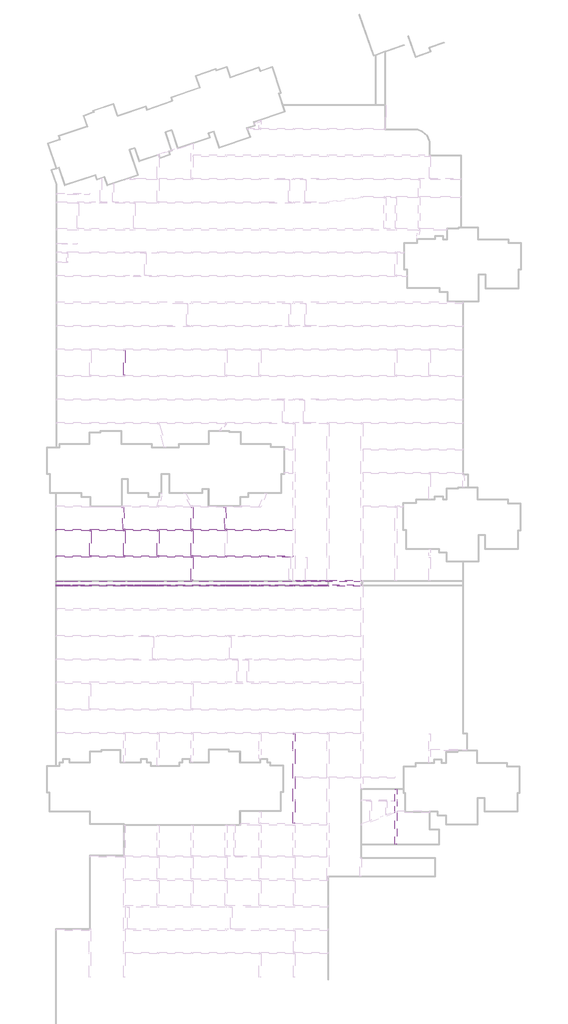
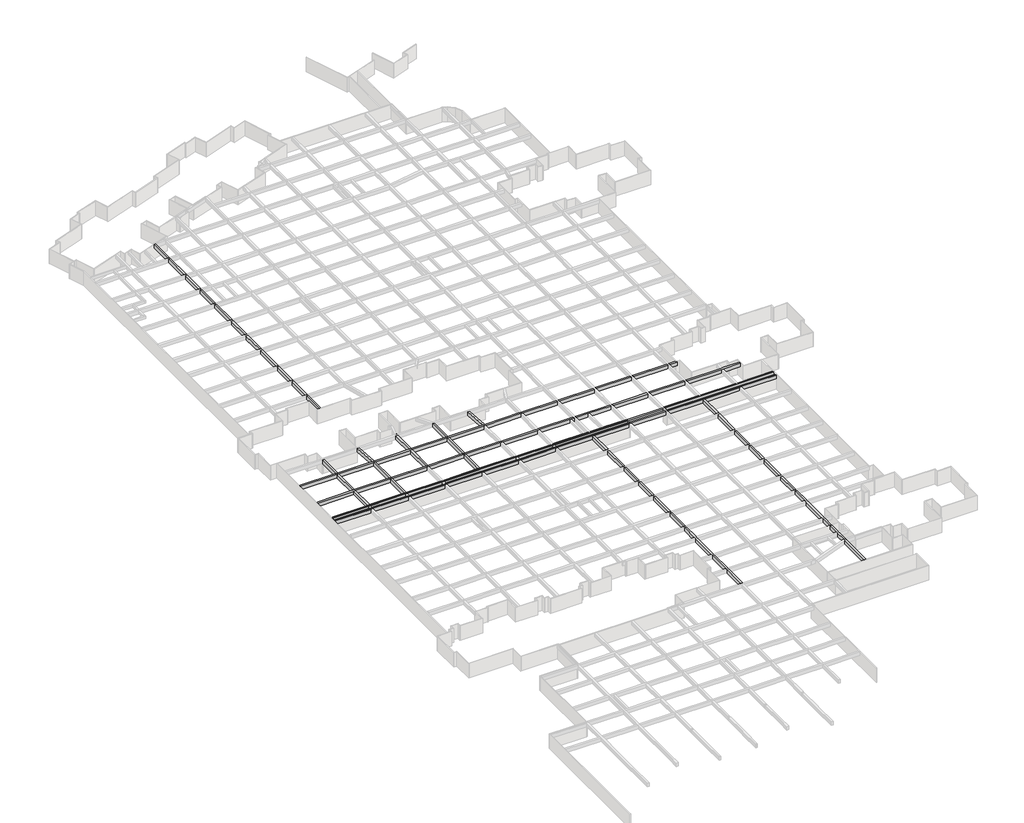
# One storey, part 10 of 14: 15 beams.
"""IFC4 building model written with IfcOpenShell, lengths in millimetres."""

from ifc_helpers import new_model, si_unit, frame, origin, place, context, project, spatial, polyline, outline, extrude, faceted_brep, element, save

model = new_model("IFC4")

# Units and contexts
model_context = context("Model", 3, world=origin())
ifc_project = project(units=[si_unit("LENGTHUNIT", "METRE", prefix="MILLI")], contexts=[model_context])

# Site, building, storey
site = spatial("IfcSite", under=ifc_project)
building = spatial("IfcBuilding", under=site)
storey = spatial("IfcBuildingStorey", under=building, Name="户型图", Elevation=0.0)

# Beams
placement = place(None, origin())
element("IfcBeam", 1, ObjectType="混凝土 - 矩形梁 : KL_beam", at=placement, inside=storey, context=model_context, shape_type="Brep", body=[
    faceted_brep([(-578267.6529954, -95855.8355501, 3300.0), (-577867.6529954, -95855.8355501, 3300.0), (-577867.6529954, -91159.4327531, 3300.0), (-578267.6529954, -91159.4327531, 3300.0), (-578267.6529954, -95855.8355501, 2500.0), (-578267.6529954, -91159.4327531, 2500.0), (-577867.6529954, -95855.8355501, 2500.0), (-577867.6529954, -91159.4327531, 2500.0)], [[[0, 1, 2, 3]], [[4, 0, 3, 5]], [[6, 4, 5, 7]], [[1, 6, 7, 2]], [[1, 0, 4, 6]], [[3, 2, 7, 5]]]),
    faceted_brep([(-578267.6529954, -33799.10215, 3300.0), (-577867.6529954, -33664.0771766, 3300.0), (-577867.6529954, -33664.0771766, 2500.0), (-578267.6529954, -33799.10215, 2500.0), (-577867.6529954, -38859.4327531, 3300.0), (-578267.6529954, -38859.4327531, 3300.0), (-578267.6529954, -38859.4327531, 2500.0), (-577867.6529954, -38859.4327531, 2500.0), (-577867.6529954, -33759.4327531, 3300.0), (-577867.6529954, -33759.4327531, 2500.0)], [[[0, 1, 2, 3]], [[4, 5, 6, 7]], [[1, 0, 5, 4, 8]], [[0, 3, 6, 5]], [[3, 2, 9, 7, 6]], [[2, 1, 8, 4, 7, 9]]]),
    faceted_brep([(-578267.6529954, -39259.4327531, 3300.0), (-577867.6529954, -39259.4327531, 3300.0), (-577867.6529954, -39259.4327531, 2500.0), (-578267.6529954, -39259.4327531, 2500.0), (-577867.6529954, -45159.4327531, 3300.0), (-578267.6529954, -45159.4327531, 3300.0), (-578267.6529954, -45159.4327531, 2500.0), (-577867.6529954, -45159.4327531, 2500.0)], [[[0, 1, 2, 3]], [[4, 5, 6, 7]], [[1, 0, 5, 4]], [[0, 3, 6, 5]], [[3, 2, 7, 6]], [[2, 1, 4, 7]]]),
    faceted_brep([(-578267.6529954, -45559.4327531, 3300.0), (-577867.6529954, -45559.4327531, 3300.0), (-577867.6529954, -45559.4327531, 2500.0), (-578267.6529954, -45559.4327531, 2500.0), (-577867.6529954, -50659.4327531, 3300.0), (-578267.6529954, -50659.4327531, 3300.0), (-578267.6529954, -50659.4327531, 2500.0), (-577867.6529954, -50659.4327531, 2500.0)], [[[0, 1, 2, 3]], [[4, 5, 6, 7]], [[1, 0, 5, 4]], [[0, 3, 6, 5]], [[3, 2, 7, 6]], [[2, 1, 4, 7]]]),
    faceted_brep([(-578267.6529954, -56559.4327531, 3300.0), (-577867.6529954, -56559.4327531, 3300.0), (-577867.6529954, -56559.4327531, 2500.0), (-578267.6529954, -56559.4327531, 2500.0), (-577867.6529954, -62459.4327531, 3300.0), (-578267.6529954, -62459.4327531, 3300.0), (-578267.6529954, -62459.4327531, 2500.0), (-577867.6529954, -62459.4327531, 2500.0)], [[[0, 1, 2, 3]], [[4, 5, 6, 7]], [[1, 0, 5, 4]], [[0, 3, 6, 5]], [[3, 2, 7, 6]], [[2, 1, 4, 7]]]),
    faceted_brep([(-577867.6529954, -56159.4327531, 3300.0), (-578267.6529954, -56159.4327531, 3300.0), (-578267.6529954, -56159.4327531, 2500.0), (-577867.6529954, -56159.4327531, 2500.0), (-577867.6529954, -51059.4327531, 3300.0), (-578267.6529954, -51059.4327531, 3300.0), (-578267.6529954, -51059.4327531, 2500.0), (-577867.6529954, -51059.4327531, 2500.0)], [[[0, 1, 2, 3]], [[1, 0, 4, 5]], [[2, 1, 5, 6]], [[3, 2, 6, 7]], [[0, 3, 7, 4]], [[5, 4, 7, 6]]]),
    faceted_brep([(-578267.6529954, -62859.4327531, 3300.0), (-577867.6529954, -62859.4327531, 3300.0), (-577867.6529954, -62859.4327531, 2500.0), (-578267.6529954, -62859.4327531, 2500.0), (-577867.6529954, -67959.4327531, 3300.0), (-578267.6529954, -67959.4327531, 3300.0), (-578267.6529954, -67959.4327531, 2500.0), (-577867.6529954, -67959.4327531, 2500.0)], [[[0, 1, 2, 3]], [[4, 5, 6, 7]], [[1, 0, 5, 4]], [[0, 3, 6, 5]], [[3, 2, 7, 6]], [[2, 1, 4, 7]]]),
    faceted_brep([(-578267.6529954, -68359.4327531, 3300.0), (-577867.6529954, -68359.4327531, 3300.0), (-577867.6529954, -68359.4327531, 2500.0), (-578267.6529954, -68359.4327531, 2500.0), (-577867.6529954, -73459.4327531, 3300.0), (-578267.6529954, -73459.4327531, 3300.0), (-578267.6529954, -73459.4327531, 2500.0), (-577867.6529954, -73459.4327531, 2500.0)], [[[0, 1, 2, 3]], [[4, 5, 6, 7]], [[1, 0, 5, 4]], [[0, 3, 6, 5]], [[3, 2, 7, 6]], [[2, 1, 4, 7]]]),
    faceted_brep([(-578267.6529954, -73859.4327531, 3300.0), (-577867.6529954, -73859.4327531, 3300.0), (-577867.6529954, -73859.4327531, 2500.0), (-578267.6529954, -73859.4327531, 2500.0), (-577867.6529954, -79759.4327531, 3300.0), (-578267.6529954, -79759.4327531, 3300.0), (-578267.6529954, -79759.4327531, 2500.0), (-577867.6529954, -79759.4327531, 2500.0)], [[[0, 1, 2, 3]], [[4, 5, 6, 7]], [[1, 0, 5, 4]], [[0, 3, 6, 5]], [[3, 2, 7, 6]], [[2, 1, 4, 7]]]),
    faceted_brep([(-578267.6529954, -80159.4327531, 3300.0), (-577867.6529954, -80159.4327531, 3300.0), (-577867.6529954, -80159.4327531, 2500.0), (-578267.6529954, -80159.4327531, 2500.0), (-577867.6529954, -85259.4327531, 3300.0), (-578267.6529954, -85259.4327531, 3300.0), (-578267.6529954, -85259.4327531, 2500.0), (-577867.6529954, -85259.4327531, 2500.0)], [[[0, 1, 2, 3]], [[4, 5, 6, 7]], [[1, 0, 5, 4]], [[0, 3, 6, 5]], [[3, 2, 7, 6]], [[2, 1, 4, 7]]]),
    faceted_brep([(-578267.6529954, -85659.4327531, 3300.0), (-577867.6529954, -85659.4327531, 3300.0), (-577867.6529954, -85659.4327531, 2500.0), (-578267.6529954, -85659.4327531, 2500.0), (-577867.6529954, -90759.4327531, 3300.0), (-578267.6529954, -90759.4327531, 3300.0), (-578267.6529954, -90759.4327531, 2500.0), (-577867.6529954, -90759.4327531, 2500.0)], [[[0, 1, 2, 3]], [[4, 5, 6, 7]], [[1, 0, 5, 4]], [[0, 3, 6, 5]], [[3, 2, 7, 6]], [[2, 1, 4, 7]]]),
])
element("IfcBeam", 2, ObjectType="混凝土 - 矩形梁 : KL_beam", at=placement, inside=storey, context=model_context, shape_type="Brep", body=[
    faceted_brep([(-512410.8523761, -116217.5126628, 3300.0), (-512410.8523761, -116097.5126628, 3300.0), (-512410.8523761, -115957.5126628, 3300.0), (-513867.6529954, -115957.5126628, 3300.0), (-513867.6529954, -116357.5126628, 3300.0), (-512290.8523761, -116357.5126628, 3300.0), (-512290.8523761, -116217.5126628, 3300.0), (-512410.8523761, -115957.5126628, 2500.0), (-513867.6529954, -115957.5126628, 2500.0), (-512410.8523761, -116217.5126628, 2500.0), (-512290.8523761, -116217.5126628, 2500.0), (-512290.8523761, -116357.5126628, 2500.0), (-513867.6529954, -116357.5126628, 2500.0)], [[[0, 1, 2, 3, 4, 5, 6]], [[2, 7, 8, 3]], [[7, 9, 10, 11, 12, 8]], [[11, 5, 4, 12]], [[5, 11, 10, 6]], [[0, 9, 7, 2, 1]], [[4, 3, 8, 12]], [[9, 0, 6, 10]]]),
    faceted_brep([(-594137.5937933, -116357.5126628, 3300.0), (-594137.5937933, -115957.5126628, 3300.0), (-594137.5937933, -115957.5126628, 2500.0), (-594137.5937933, -116357.5126628, 2500.0), (-538267.6529954, -115957.5126628, 3300.0), (-538267.6529954, -116357.5126628, 3300.0), (-538267.6529954, -116357.5126628, 2500.0), (-538267.6529954, -115957.5126628, 2500.0), (-586231.2602569, -116357.5126628, 3300.0), (-585831.2602569, -116357.5126628, 3300.0), (-578267.6529954, -116357.5126628, 3300.0), (-577867.6529954, -116357.5126628, 3300.0), (-570267.6529954, -116357.5126628, 3300.0), (-569867.6529954, -116357.5126628, 3300.0), (-562267.6529954, -116357.5126628, 3300.0), (-561867.6529954, -116357.5126628, 3300.0), (-554267.6529954, -116357.5126628, 3300.0), (-553867.6529954, -116357.5126628, 3300.0), (-546267.6529954, -116357.5126628, 3300.0), (-545867.6529954, -116357.5126628, 3300.0), (-545867.6529954, -115957.5126628, 3300.0), (-546267.6529954, -115957.5126628, 3300.0), (-553881.1620009, -115957.5126628, 3300.0), (-554282.1387601, -115957.5126628, 3300.0), (-561867.6529954, -115957.5126628, 3300.0), (-562267.6529954, -115957.5126628, 3300.0), (-569867.6529954, -115957.5126628, 3300.0), (-570267.6529954, -115957.5126628, 3300.0), (-577881.1499782, -115957.5126628, 3300.0), (-578282.1267374, -115957.5126628, 3300.0), (-585831.2602569, -115957.5126628, 3300.0), (-586231.2602569, -115957.5126628, 3300.0), (-545867.6529954, -115957.5126628, 2500.0), (-546267.6529954, -115957.5126628, 2500.0), (-553881.1620009, -115957.5126628, 2500.0), (-554282.1387601, -115957.5126628, 2500.0), (-561867.6529954, -115957.5126628, 2500.0), (-562267.6529954, -115957.5126628, 2500.0), (-569867.6529954, -115957.5126628, 2500.0), (-570267.6529954, -115957.5126628, 2500.0), (-577881.1499782, -115957.5126628, 2500.0), (-578282.1267374, -115957.5126628, 2500.0), (-585831.2602569, -115957.5126628, 2500.0), (-586231.2602569, -115957.5126628, 2500.0), (-545867.6529954, -116357.5126628, 2500.0), (-546267.6529954, -116357.5126628, 2500.0), (-553867.6529954, -116357.5126628, 2500.0), (-554267.6529954, -116357.5126628, 2500.0), (-561867.6529954, -116357.5126628, 2500.0), (-562267.6529954, -116357.5126628, 2500.0), (-569867.6529954, -116357.5126628, 2500.0), (-570267.6529954, -116357.5126628, 2500.0), (-577867.6529954, -116357.5126628, 2500.0), (-578267.6529954, -116357.5126628, 2500.0), (-585831.2602569, -116357.5126628, 2500.0), (-586231.2602569, -116357.5126628, 2500.0)], [[[0, 1, 2, 3]], [[4, 5, 6, 7]], [[1, 0, 8, 9, 10, 11, 12, 13, 14, 15, 16, 17, 18, 19, 5, 4, 20, 21, 22, 23, 24, 25, 26, 27, 28, 29, 30, 31]], [[2, 1, 31, 30, 29, 28, 27, 26, 25, 24, 23, 22, 21, 20, 4, 7, 32, 33, 34, 35, 36, 37, 38, 39, 40, 41, 42, 43]], [[3, 2, 43, 42, 41, 40, 39, 38, 37, 36, 35, 34, 33, 32, 7, 6, 44, 45, 46, 47, 48, 49, 50, 51, 52, 53, 54, 55]], [[0, 3, 55, 54, 53, 52, 51, 50, 49, 48, 47, 46, 45, 44, 6, 5, 19, 18, 17, 16, 15, 14, 13, 12, 11, 10, 9, 8]]]),
    faceted_brep([(-537867.6529954, -116357.5126628, 3300.0), (-537867.6529954, -115957.5126628, 3300.0), (-537867.6529954, -115957.5126628, 2500.0), (-537867.6529954, -116357.5126628, 2500.0), (-530267.6529954, -115957.5126628, 3300.0), (-530267.6529954, -116357.5126628, 3300.0), (-530267.6529954, -116357.5126628, 2500.0), (-530267.6529954, -115957.5126628, 2500.0)], [[[0, 1, 2, 3]], [[4, 5, 6, 7]], [[1, 0, 5, 4]], [[2, 1, 4, 7]], [[3, 2, 7, 6]], [[0, 3, 6, 5]]]),
    faceted_brep([(-529867.6529954, -116357.5126628, 3300.0), (-529867.6529954, -115957.5126628, 3300.0), (-529867.6529954, -115957.5126628, 2500.0), (-529867.6529954, -116357.5126628, 2500.0), (-522267.6529954, -115957.5126628, 3300.0), (-522267.6529954, -116357.5126628, 3300.0), (-522267.6529954, -116357.5126628, 2500.0), (-522267.6529954, -115957.5126628, 2500.0)], [[[0, 1, 2, 3]], [[4, 5, 6, 7]], [[1, 0, 5, 4]], [[2, 1, 4, 7]], [[3, 2, 7, 6]], [[0, 3, 6, 5]]]),
    faceted_brep([(-521867.6529954, -116357.5126628, 3300.0), (-521867.6529954, -115957.5126628, 3300.0), (-521867.6529954, -115957.5126628, 2500.0), (-521867.6529954, -116357.5126628, 2500.0), (-514267.6529954, -115957.5126628, 3300.0), (-514267.6529954, -116357.5126628, 3300.0), (-514267.6529954, -116357.5126628, 2500.0), (-514267.6529954, -115957.5126628, 2500.0)], [[[0, 1, 2, 3]], [[4, 5, 6, 7]], [[1, 0, 5, 4]], [[2, 1, 4, 7]], [[3, 2, 7, 6]], [[0, 3, 6, 5]]]),
])
element("IfcBeam", 3, ObjectType="混凝土 - 矩形梁 : KL_beam", at=placement, inside=storey, context=model_context, shape_type="Brep", body=[
    faceted_brep([(-594137.5937933, -122259.4327531, 3300.0), (-594137.5937933, -122659.4327531, 3300.0), (-586231.2602569, -122659.4327531, 3300.0), (-585831.2602569, -122659.4327531, 3300.0), (-578267.6529954, -122659.4327531, 3300.0), (-577867.6529954, -122659.4327531, 3300.0), (-570267.6529954, -122659.4327531, 3300.0), (-569867.6529954, -122659.4327531, 3300.0), (-562267.6529954, -122659.4327531, 3300.0), (-561867.6529954, -122659.4327531, 3300.0), (-554267.6529954, -122659.4327531, 3300.0), (-553867.6529954, -122659.4327531, 3300.0), (-546267.6529954, -122659.4327531, 3300.0), (-545867.6529954, -122659.4327531, 3300.0), (-539217.6529954, -122659.4327531, 3300.0), (-538917.6529954, -122659.4327531, 3300.0), (-538267.6529954, -122659.4327531, 3300.0), (-538267.6529954, -122259.4327531, 3300.0), (-545867.6529954, -122259.4327531, 3300.0), (-546267.6529954, -122259.4327531, 3300.0), (-553867.6529954, -122259.4327531, 3300.0), (-554267.6529954, -122259.4327531, 3300.0), (-561867.6529954, -122259.4327531, 3300.0), (-562267.6529954, -122259.4327531, 3300.0), (-569867.6529954, -122259.4327531, 3300.0), (-570267.6529954, -122259.4327531, 3300.0), (-577867.6529954, -122259.4327531, 3300.0), (-578267.6529954, -122259.4327531, 3300.0), (-585831.2602569, -122259.4327531, 3300.0), (-586231.2602569, -122259.4327531, 3300.0), (-594137.5937933, -122659.4327531, 2500.0), (-586231.2602569, -122659.4327531, 2500.0), (-585831.2602569, -122659.4327531, 2500.0), (-578267.6529954, -122659.4327531, 2500.0), (-577867.6529954, -122659.4327531, 2500.0), (-570267.6529954, -122659.4327531, 2500.0), (-569867.6529954, -122659.4327531, 2500.0), (-562267.6529954, -122659.4327531, 2500.0), (-561867.6529954, -122659.4327531, 2500.0), (-554267.6529954, -122659.4327531, 2500.0), (-553867.6529954, -122659.4327531, 2500.0), (-546267.6529954, -122659.4327531, 2500.0), (-545867.6529954, -122659.4327531, 2500.0), (-538267.6529954, -122659.4327531, 2500.0), (-594137.5937933, -122259.4327531, 2500.0), (-586231.2602569, -122259.4327531, 2500.0), (-585831.2602569, -122259.4327531, 2500.0), (-578267.6529954, -122259.4327531, 2500.0), (-577867.6529954, -122259.4327531, 2500.0), (-570267.6529954, -122259.4327531, 2500.0), (-569867.6529954, -122259.4327531, 2500.0), (-562267.6529954, -122259.4327531, 2500.0), (-561867.6529954, -122259.4327531, 2500.0), (-554267.6529954, -122259.4327531, 2500.0), (-553867.6529954, -122259.4327531, 2500.0), (-546267.6529954, -122259.4327531, 2500.0), (-545867.6529954, -122259.4327531, 2500.0), (-538267.6529954, -122259.4327531, 2500.0)], [[[0, 1, 2, 3, 4, 5, 6, 7, 8, 9, 10, 11, 12, 13, 14, 15, 16, 17, 18, 19, 20, 21, 22, 23, 24, 25, 26, 27, 28, 29]], [[1, 30, 31, 32, 33, 34, 35, 36, 37, 38, 39, 40, 41, 42, 43, 16, 15, 14, 13, 12, 11, 10, 9, 8, 7, 6, 5, 4, 3, 2]], [[30, 44, 45, 46, 47, 48, 49, 50, 51, 52, 53, 54, 55, 56, 57, 43, 42, 41, 40, 39, 38, 37, 36, 35, 34, 33, 32, 31]], [[44, 0, 29, 28, 27, 26, 25, 24, 23, 22, 21, 20, 19, 18, 17, 57, 56, 55, 54, 53, 52, 51, 50, 49, 48, 47, 46, 45]], [[1, 0, 44, 30]], [[17, 16, 43, 57]]]),
    faceted_brep([(-502127.6529954, -122259.4327531, 3300.0), (-502127.6529954, -122659.4327531, 3300.0), (-502127.6529954, -122659.4327531, 2500.0), (-502127.6529954, -122259.4327531, 2500.0), (-505867.6529954, -122259.4327531, 3300.0), (-506267.6529954, -122259.4327531, 3300.0), (-513867.6529954, -122259.4327531, 3300.0), (-513867.6529954, -122659.4327531, 3300.0), (-506267.6529954, -122659.4327531, 3300.0), (-505867.6529954, -122659.4327531, 3300.0), (-513867.6529954, -122659.4327531, 2500.0), (-506267.6529954, -122659.4327531, 2500.0), (-505867.6529954, -122659.4327531, 2500.0), (-513867.6529954, -122259.4327531, 2500.0), (-506267.6529954, -122259.4327531, 2500.0), (-505867.6529954, -122259.4327531, 2500.0)], [[[0, 1, 2, 3]], [[1, 0, 4, 5, 6, 7, 8, 9]], [[2, 1, 9, 8, 7, 10, 11, 12]], [[3, 2, 12, 11, 10, 13, 14, 15]], [[0, 3, 15, 14, 13, 6, 5, 4]], [[7, 6, 13, 10]]]),
    faceted_brep([(-537867.6529954, -122659.4327531, 3300.0), (-537867.6529954, -122259.4327531, 3300.0), (-537867.6529954, -122259.4327531, 2500.0), (-537867.6529954, -122659.4327531, 2500.0), (-530267.6529954, -122259.4327531, 3300.0), (-530267.6529954, -122659.4327531, 3300.0), (-530267.6529954, -122659.4327531, 2500.0), (-530267.6529954, -122259.4327531, 2500.0), (-535317.6529954, -122659.4327531, 3300.0), (-535017.6529954, -122659.4327531, 3300.0)], [[[0, 1, 2, 3]], [[4, 5, 6, 7]], [[1, 0, 8, 9, 5, 4]], [[0, 3, 6, 5, 9, 8]], [[3, 2, 7, 6]], [[2, 1, 4, 7]]]),
    faceted_brep([(-529867.6529954, -122259.4327531, 3300.0), (-529867.6529954, -122659.4327531, 3300.0), (-522267.6529954, -122659.4327531, 3300.0), (-522267.6529954, -122259.4327531, 3300.0), (-529867.6529954, -122659.4327531, 2500.0), (-522267.6529954, -122659.4327531, 2500.0), (-529867.6529954, -122259.4327531, 2500.0), (-522267.6529954, -122259.4327531, 2500.0)], [[[0, 1, 2, 3]], [[1, 4, 5, 2]], [[4, 6, 7, 5]], [[6, 0, 3, 7]], [[1, 0, 6, 4]], [[3, 2, 5, 7]]]),
    faceted_brep([(-521867.6529954, -122659.4327531, 3300.0), (-521867.6529954, -122259.4327531, 3300.0), (-521867.6529954, -122259.4327531, 2500.0), (-521867.6529954, -122659.4327531, 2500.0), (-514267.6529954, -122259.4327531, 3300.0), (-514267.6529954, -122659.4327531, 3300.0), (-514267.6529954, -122659.4327531, 2500.0), (-514267.6529954, -122259.4327531, 2500.0)], [[[0, 1, 2, 3]], [[4, 5, 6, 7]], [[1, 0, 5, 4]], [[0, 3, 6, 5]], [[3, 2, 7, 6]], [[2, 1, 4, 7]]]),
])
element("IfcBeam", 4, ObjectType="混凝土 - 矩形梁 : KL_beam", at=placement, inside=storey, context=model_context, shape_type="Brep", body=[
    faceted_brep([(-521867.6529954, -128359.4327532, 3300.0), (-498227.6529954, -128359.4327532, 3300.0), (-498227.6529954, -128219.4327532, 3300.0), (-521867.6529954, -128219.4327532, 3300.0), (-498227.6529954, -128359.4327532, 2500.0), (-521867.6529954, -128359.4327532, 2500.0), (-498227.6529954, -128219.4327532, 2500.0), (-521867.6529954, -128219.4327532, 2500.0)], [[[0, 1, 2, 3]], [[4, 1, 0, 5]], [[2, 6, 7, 3]], [[4, 5, 7, 6]], [[1, 4, 6, 2]], [[5, 0, 3, 7]]]),
    faceted_brep([(-498227.6529954, -127959.4327532, 3300.0), (-498227.6529954, -127959.4327532, 2500.0), (-505867.6529954, -127959.4327532, 2500.0), (-505867.6529954, -127959.4327532, 3300.0), (-498227.6529954, -128099.4327532, 3300.0), (-498227.6529954, -128099.4327532, 2500.0), (-505867.6529954, -128099.4327532, 2500.0), (-505867.6529954, -128099.4327532, 3300.0)], [[[0, 1, 2, 3]], [[1, 0, 4, 5]], [[3, 2, 6, 7]], [[4, 7, 6, 5]], [[0, 3, 7, 4]], [[2, 1, 5, 6]]]),
    faceted_brep([(-521867.6529954, -127959.4327532, 2500.0), (-514267.6529954, -127959.4327532, 2500.0), (-514267.6529954, -128099.4327532, 2500.0), (-521867.6529954, -128099.4327532, 2500.0), (-521867.6529954, -127959.4327532, 3300.0), (-521867.6529954, -128099.4327532, 3300.0), (-514267.6529954, -127959.4327532, 3300.0), (-514267.6529954, -128099.4327532, 3300.0)], [[[0, 1, 2, 3]], [[4, 0, 3, 5]], [[1, 6, 7, 2]], [[0, 4, 6, 1]], [[6, 4, 5, 7]], [[7, 5, 3, 2]]]),
    faceted_brep([(-594137.5937933, -128359.4327532, 2500.0), (-594137.5937933, -128359.4327532, 3300.0), (-594137.5937933, -128219.4327532, 3300.0), (-594137.5937933, -128219.4327532, 2500.0), (-537867.6529954, -127959.4327532, 3300.0), (-537867.6529954, -127959.4327532, 2500.0), (-537867.6529954, -128099.4327532, 2500.0), (-537867.6529954, -128099.4327532, 3300.0), (-530067.6731545, -128219.4327532, 3300.0), (-530067.6731545, -128219.4327532, 2500.0), (-522267.6529954, -127959.4327532, 3300.0), (-522267.6529954, -128359.4327532, 3300.0), (-522267.6529954, -128359.4327532, 2500.0), (-522267.6529954, -127959.4327532, 2500.0), (-586331.2602569, -128359.4327532, 3300.0), (-585931.2602569, -128359.4327532, 3300.0), (-578267.6529954, -128359.4327532, 3300.0), (-577867.6529954, -128359.4327532, 3300.0), (-570267.6529954, -128359.4327532, 3300.0), (-569867.6529954, -128359.4327532, 3300.0), (-554267.6529954, -128359.4327532, 3300.0), (-553867.6529954, -128359.4327532, 3300.0), (-546267.6529954, -128359.4327532, 3300.0), (-545867.6529954, -128359.4327532, 3300.0), (-529867.6529954, -127959.4327532, 3300.0), (-530267.6529954, -127959.4327532, 3300.0), (-535017.6529954, -127959.4327532, 3300.0), (-535317.6529954, -127959.4327532, 3300.0), (-530067.6731545, -128099.4327532, 3300.0), (-529867.6529954, -127959.4327532, 2500.0), (-530267.6529954, -127959.4327532, 2500.0), (-586331.2602569, -128359.4327532, 2500.0), (-585931.2602569, -128359.4327532, 2500.0), (-578267.6529954, -128359.4327532, 2500.0), (-577867.6529954, -128359.4327532, 2500.0), (-570267.6529954, -128359.4327532, 2500.0), (-569867.6529954, -128359.4327532, 2500.0), (-554267.6529954, -128359.4327532, 2500.0), (-553867.6529954, -128359.4327532, 2500.0), (-546267.6529954, -128359.4327532, 2500.0), (-545867.6529954, -128359.4327532, 2500.0), (-530067.6731545, -128099.4327532, 2500.0)], [[[0, 1, 2, 3]], [[4, 5, 6, 7]], [[8, 9, 3, 2]], [[10, 11, 12, 13]], [[1, 14, 15, 16, 17, 18, 19, 20, 21, 22, 23, 11, 10, 24, 25, 26, 27, 4, 7, 28, 8, 2]], [[5, 4, 27, 26, 25, 24, 10, 13, 29, 30]], [[1, 0, 31, 32, 33, 34, 35, 36, 37, 38, 39, 40, 12, 11, 23, 22, 21, 20, 19, 18, 17, 16, 15, 14]], [[41, 28, 7, 6]], [[9, 8, 28, 41]], [[5, 30, 29, 13, 12, 40, 39, 38, 37, 36, 35, 34, 33, 32, 31, 0, 3, 9, 41, 6]]]),
    faceted_brep([(-538267.6529954, -127959.4327532, 2500.0), (-538267.6529954, -127959.4327532, 3300.0), (-538267.6529954, -128099.4327532, 3300.0), (-538267.6529954, -128099.4327532, 2500.0), (-594137.5937933, -127959.4327532, 2500.0), (-594137.5937933, -127959.4327532, 3300.0), (-586231.2602569, -127959.4327532, 3300.0), (-585831.2602569, -127959.4327532, 3300.0), (-578267.6529954, -127959.4327532, 3300.0), (-577867.6529954, -127959.4327532, 3300.0), (-570267.6529954, -127959.4327532, 3300.0), (-569867.6529954, -127959.4327532, 3300.0), (-562267.6529954, -127959.4327532, 3300.0), (-561867.6529954, -127959.4327532, 3300.0), (-554267.6529954, -127959.4327532, 3300.0), (-553867.6529954, -127959.4327532, 3300.0), (-546267.6529954, -127959.4327532, 3300.0), (-545867.6529954, -127959.4327532, 3300.0), (-545867.6529954, -127959.4327532, 2500.0), (-546267.6529954, -127959.4327532, 2500.0), (-553867.6529954, -127959.4327532, 2500.0), (-554267.6529954, -127959.4327532, 2500.0), (-561867.6529954, -127959.4327532, 2500.0), (-562267.6529954, -127959.4327532, 2500.0), (-569867.6529954, -127959.4327532, 2500.0), (-570267.6529954, -127959.4327532, 2500.0), (-577867.6529954, -127959.4327532, 2500.0), (-578267.6529954, -127959.4327532, 2500.0), (-585831.2602569, -127959.4327532, 2500.0), (-586231.2602569, -127959.4327532, 2500.0), (-594137.5937933, -128099.4327532, 2500.0), (-594137.5937933, -128099.4327532, 3300.0)], [[[0, 1, 2, 3]], [[4, 5, 6, 7, 8, 9, 10, 11, 12, 13, 14, 15, 16, 17, 1, 0, 18, 19, 20, 21, 22, 23, 24, 25, 26, 27, 28, 29]], [[4, 29, 28, 27, 26, 25, 24, 23, 22, 21, 20, 19, 18, 0, 3, 30]], [[5, 4, 30, 31]], [[1, 17, 16, 15, 14, 13, 12, 11, 10, 9, 8, 7, 6, 5, 31, 2]], [[31, 30, 3, 2]]]),
    faceted_brep([(-513867.6529954, -127959.4327532, 3300.0), (-513867.6529954, -127959.4327532, 2500.0), (-513867.6529954, -128099.4327532, 2500.0), (-513867.6529954, -128099.4327532, 3300.0), (-506267.6529954, -127959.4327532, 2500.0), (-506267.6529954, -127959.4327532, 3300.0), (-506267.6529954, -128099.4327532, 3300.0), (-506267.6529954, -128099.4327532, 2500.0)], [[[0, 1, 2, 3]], [[4, 5, 6, 7]], [[1, 0, 5, 4]], [[5, 0, 3, 6]], [[1, 4, 7, 2]], [[6, 3, 2, 7]]]),
])
element("IfcBeam", 5, ObjectType="混凝土 - 矩形梁 : KL_beam", at=placement, inside=storey, context=model_context, shape_type="Brep", body=[
    faceted_brep([(-522267.6529954, -129034.4327531, 3300.0), (-545867.6529954, -129034.4327531, 3300.0), (-546267.6529954, -129034.4327531, 3300.0), (-553867.6529954, -129034.4327531, 3300.0), (-554267.6529954, -129034.4327531, 3300.0), (-569867.6529954, -129034.4327531, 3300.0), (-570267.6529954, -129034.4327531, 3300.0), (-577867.6529954, -129034.4327531, 3300.0), (-578267.6529954, -129034.4327531, 3300.0), (-585931.2602569, -129034.4327531, 3300.0), (-586331.2602569, -129034.4327531, 3300.0), (-594137.5937933, -129034.4327531, 3300.0), (-594137.5937933, -129174.4327531, 3300.0), (-530067.6731545, -129174.4327531, 3300.0), (-530067.6731545, -129294.4327531, 3300.0), (-594137.5937933, -129294.4327531, 3300.0), (-594137.5937933, -129434.4327531, 3300.0), (-586331.2602569, -129434.4327531, 3300.0), (-585931.2602569, -129434.4327531, 3300.0), (-578267.6529954, -129434.4327531, 3300.0), (-577867.6529954, -129434.4327531, 3300.0), (-570267.6529954, -129434.4327531, 3300.0), (-569867.6529954, -129434.4327531, 3300.0), (-562267.6529954, -129434.4327531, 3300.0), (-561867.6529954, -129434.4327531, 3300.0), (-554267.6529954, -129434.4327531, 3300.0), (-553867.6529954, -129434.4327531, 3300.0), (-546267.6529954, -129434.4327531, 3300.0), (-545867.6529954, -129434.4327531, 3300.0), (-538267.6529954, -129434.4327531, 3300.0), (-537867.6529954, -129434.4327531, 3300.0), (-530267.6529954, -129434.4327531, 3300.0), (-529867.6529954, -129434.4327531, 3300.0), (-522267.6529954, -129434.4327531, 3300.0), (-594137.5937933, -129434.4327531, 2500.0), (-586331.2602569, -129434.4327531, 2500.0), (-585931.2602569, -129434.4327531, 2500.0), (-578267.6529954, -129434.4327531, 2500.0), (-577867.6529954, -129434.4327531, 2500.0), (-570267.6529954, -129434.4327531, 2500.0), (-569867.6529954, -129434.4327531, 2500.0), (-562267.6529954, -129434.4327531, 2500.0), (-561867.6529954, -129434.4327531, 2500.0), (-554267.6529954, -129434.4327531, 2500.0), (-553867.6529954, -129434.4327531, 2500.0), (-546267.6529954, -129434.4327531, 2500.0), (-545867.6529954, -129434.4327531, 2500.0), (-538267.6529954, -129434.4327531, 2500.0), (-537867.6529954, -129434.4327531, 2500.0), (-530267.6529954, -129434.4327531, 2500.0), (-529867.6529954, -129434.4327531, 2500.0), (-522267.6529954, -129434.4327531, 2500.0), (-594137.5937933, -129294.4327531, 2500.0), (-530067.6731545, -129294.4327531, 2500.0), (-530067.6731545, -129174.4327531, 2500.0), (-594137.5937933, -129174.4327531, 2500.0), (-594137.5937933, -129034.4327531, 2500.0), (-586331.2602569, -129034.4327531, 2500.0), (-585931.2602569, -129034.4327531, 2500.0), (-578267.6529954, -129034.4327531, 2500.0), (-577867.6529954, -129034.4327531, 2500.0), (-570267.6529954, -129034.4327531, 2500.0), (-569867.6529954, -129034.4327531, 2500.0), (-554267.6529954, -129034.4327531, 2500.0), (-553867.6529954, -129034.4327531, 2500.0), (-546267.6529954, -129034.4327531, 2500.0), (-545867.6529954, -129034.4327531, 2500.0), (-522267.6529954, -129034.4327531, 2500.0)], [[[0, 1, 2, 3, 4, 5, 6, 7, 8, 9, 10, 11, 12, 13, 14, 15, 16, 17, 18, 19, 20, 21, 22, 23, 24, 25, 26, 27, 28, 29, 30, 31, 32, 33]], [[16, 34, 35, 36, 37, 38, 39, 40, 41, 42, 43, 44, 45, 46, 47, 48, 49, 50, 51, 33, 32, 31, 30, 29, 28, 27, 26, 25, 24, 23, 22, 21, 20, 19, 18, 17]], [[51, 50, 49, 48, 47, 46, 45, 44, 43, 42, 41, 40, 39, 38, 37, 36, 35, 34, 52, 53, 54, 55, 56, 57, 58, 59, 60, 61, 62, 63, 64, 65, 66, 67]], [[56, 11, 10, 9, 8, 7, 6, 5, 4, 3, 2, 1, 0, 67, 66, 65, 64, 63, 62, 61, 60, 59, 58, 57]], [[34, 16, 15, 52]], [[0, 33, 51, 67]], [[54, 13, 12, 55]], [[14, 53, 52, 15]], [[13, 54, 53, 14]], [[11, 56, 55, 12]]]),
    faceted_brep([(-498227.6529954, -129034.4327531, 2500.0), (-498227.6529954, -129034.4327531, 3300.0), (-498227.6529954, -129174.4327531, 3300.0), (-498227.6529954, -129174.4327531, 2500.0), (-521867.6529954, -129034.4327531, 3300.0), (-521867.6529954, -129174.4327531, 3300.0), (-521867.6529954, -129034.4327531, 2500.0), (-521867.6529954, -129174.4327531, 2500.0)], [[[0, 1, 2, 3]], [[1, 4, 5, 2]], [[1, 0, 6, 4]], [[3, 2, 5, 7]], [[4, 6, 7, 5]], [[6, 0, 3, 7]]]),
    faceted_brep([(-521867.6529954, -129434.4327531, 2500.0), (-521867.6529954, -129434.4327531, 3300.0), (-521867.6529954, -129294.4327531, 3300.0), (-521867.6529954, -129294.4327531, 2500.0), (-498227.6529954, -129434.4327531, 2500.0), (-498227.6529954, -129434.4327531, 3300.0), (-505867.6529954, -129434.4327531, 3300.0), (-506267.6529954, -129434.4327531, 3300.0), (-513867.6529954, -129434.4327531, 3300.0), (-514267.6529954, -129434.4327531, 3300.0), (-514267.6529954, -129434.4327531, 2500.0), (-513867.6529954, -129434.4327531, 2500.0), (-506267.6529954, -129434.4327531, 2500.0), (-505867.6529954, -129434.4327531, 2500.0), (-498227.6529954, -129294.4327531, 2500.0), (-498227.6529954, -129294.4327531, 3300.0)], [[[0, 1, 2, 3]], [[4, 5, 6, 7, 8, 9, 1, 0, 10, 11, 12, 13]], [[4, 13, 12, 11, 10, 0, 3, 14]], [[15, 14, 3, 2]], [[5, 4, 14, 15]], [[1, 9, 8, 7, 6, 5, 15, 2]]]),
])
element("IfcBeam", 6, ObjectType="混凝土 - 矩形梁 : KL_beam", at=placement, inside=storey, context=model_context, shape_type="SweptSolid", body=[
    extrude(outline(polyline([(-553881.1620009, -115957.5126628), (-554282.1387601, -115957.5126628), (-554638.6312353, -110859.4327531), (-554237.654476, -110859.4327531), (-553881.1620009, -115957.5126628)])), frame((0.0, 0.0, 2500.0), z_axis=(0.0, 0.0, 1.0), x_axis=(1.0, 0.0, 0.0)), (0.0, 0.0, 1.0), 800.0),
])
element("IfcBeam", 7, ObjectType="混凝土 - 矩形梁 : KL_beam", at=placement, inside=storey, context=model_context, shape_type="SweptSolid", body=[
    extrude(outline(polyline([(-562267.6529954, -116357.5126628), (-561867.6529954, -116357.5126628), (-561867.6529954, -122259.4327531), (-562267.6529954, -122259.4327531), (-562267.6529954, -116357.5126628)])), frame((0.0, 0.0, 2500.0), z_axis=(0.0, 0.0, 1.0), x_axis=(1.0, 0.0, 0.0)), (0.0, 0.0, 1.0), 800.0),
])
element("IfcBeam", 8, ObjectType="混凝土 - 矩形梁 : KL_beam", at=placement, inside=storey, context=model_context, shape_type="SweptSolid", body=[
    extrude(outline(polyline([(-561867.6529954, -115957.5126628), (-562267.6529954, -115957.5126628), (-562267.6529954, -110859.4327531), (-561867.6529954, -110859.4327531), (-561867.6529954, -115957.5126628)])), frame((0.0, 0.0, 2500.0), z_axis=(0.0, 0.0, 1.0), x_axis=(1.0, 0.0, 0.0)), (0.0, 0.0, 1.0), 800.0),
])
element("IfcBeam", 9, ObjectType="混凝土 - 矩形梁 : KL_beam", at=placement, inside=storey, context=model_context, shape_type="Brep", body=[
    faceted_brep([(-569872.5620528, -110459.4327531, 3300.0), (-569867.6529954, -110459.4327531, 3300.0), (-569867.6529954, -110440.9518528, 3300.0), (-569867.6529954, -110459.4327531, 2500.0), (-569867.6529954, -110440.9518528, 2500.0), (-569872.5620528, -110459.4327531, 2500.0)], [[[0, 1, 2]], [[1, 3, 4, 2]], [[4, 3, 5]], [[3, 1, 0, 5]], [[0, 2, 4, 5]]]),
    faceted_brep([(-569867.6529954, -122259.4327531, 3300.0), (-570267.6529954, -122259.4327531, 3300.0), (-570267.6529954, -122259.4327531, 2500.0), (-569867.6529954, -122259.4327531, 2500.0), (-570267.6529954, -116357.5126628, 3300.0), (-569867.6529954, -116357.5126628, 3300.0), (-569867.6529954, -116357.5126628, 2500.0), (-570267.6529954, -116357.5126628, 2500.0)], [[[0, 1, 2, 3]], [[4, 5, 6, 7]], [[1, 0, 5, 4]], [[0, 3, 6, 5]], [[3, 2, 7, 6]], [[2, 1, 4, 7]]]),
    faceted_brep([(-569867.6529954, -115957.5126628, 3300.0), (-570267.6529954, -115957.5126628, 3300.0), (-570267.6529954, -115957.5126628, 2500.0), (-569867.6529954, -115957.5126628, 2500.0), (-569867.6529954, -110859.4327531, 3300.0), (-569867.6529954, -110859.4327531, 2500.0), (-569978.8135288, -110859.4327531, 2500.0), (-570267.6529954, -110859.4327531, 2500.0), (-570267.6529954, -110859.4327531, 3300.0), (-569978.8135288, -110859.4327531, 3300.0)], [[[0, 1, 2, 3]], [[4, 5, 6, 7, 8, 9]], [[1, 0, 4, 9, 8]], [[0, 3, 5, 4]], [[3, 2, 7, 6, 5]], [[2, 1, 8, 7]]]),
])
element("IfcBeam", 10, ObjectType="混凝土 - 矩形梁 : KL_beam", at=placement, inside=storey, context=model_context, shape_type="SweptSolid", body=[
    extrude(outline(polyline([(-577867.6529954, -127959.4327532), (-578267.6529954, -127959.4327532), (-578267.6529954, -122659.4327531), (-577867.6529954, -122659.4327531), (-577867.6529954, -127959.4327532)])), frame((0.0, 0.0, 2500.0), z_axis=(0.0, 0.0, 1.0), x_axis=(1.0, 0.0, 0.0)), (0.0, 0.0, 1.0), 800.0),
    extrude(outline(polyline([(-578267.6529954, -116357.5126628), (-577867.6529954, -116357.5126628), (-577867.6529954, -122259.4327531), (-578267.6529954, -122259.4327531), (-578267.6529954, -116357.5126628)])), frame((0.0, 0.0, 2500.0), z_axis=(0.0, 0.0, 1.0), x_axis=(1.0, 0.0, 0.0)), (0.0, 0.0, 1.0), 800.0),
])
element("IfcBeam", 11, ObjectType="混凝土 - 矩形梁 : KL_beam", at=placement, inside=storey, context=model_context, shape_type="SweptSolid", body=[
    extrude(outline(polyline([(-577881.1499782, -115957.5126628), (-578282.1267374, -115957.5126628), (-578638.6192125, -110859.4327531), (-578237.6424533, -110859.4327531), (-577881.1499782, -115957.5126628)])), frame((0.0, 0.0, 2500.0), z_axis=(0.0, 0.0, 1.0), x_axis=(1.0, 0.0, 0.0)), (0.0, 0.0, 1.0), 800.0),
])
element("IfcBeam", 12, ObjectType="混凝土 - 矩形梁 : KL_beam", at=placement, inside=storey, context=model_context, shape_type="SweptSolid", body=[
    extrude(outline(polyline([(-586231.2602569, -110859.4327531), (-585831.2602569, -110859.4327531), (-585831.2602569, -115957.5126628), (-586231.2602569, -115957.5126628), (-586231.2602569, -110859.4327531)])), frame((0.0, 0.0, 2500.0), z_axis=(0.0, 0.0, 1.0), x_axis=(1.0, 0.0, 0.0)), (0.0, 0.0, 1.0), 800.0),
    extrude(outline(polyline([(-585831.2602569, -127959.4327532), (-586231.2602569, -127959.4327532), (-586231.2602569, -122659.4327531), (-585831.2602569, -122659.4327531), (-585831.2602569, -127959.4327532)])), frame((0.0, 0.0, 2500.0), z_axis=(0.0, 0.0, 1.0), x_axis=(1.0, 0.0, 0.0)), (0.0, 0.0, 1.0), 800.0),
    extrude(outline(polyline([(-586231.2602569, -116357.5126628), (-585831.2602569, -116357.5126628), (-585831.2602569, -122259.4327531), (-586231.2602569, -122259.4327531), (-586231.2602569, -116357.5126628)])), frame((0.0, 0.0, 2500.0), z_axis=(0.0, 0.0, 1.0), x_axis=(1.0, 0.0, 0.0)), (0.0, 0.0, 1.0), 800.0),
])
element("IfcBeam", 13, ObjectType="混凝土 - 矩形梁 : KL_beam", at=placement, inside=storey, context=model_context, shape_type="SweptSolid", body=[
    extrude(outline(polyline([(-562267.6529954, -122659.4327531), (-561867.6529954, -122659.4327531), (-561867.6529954, -127959.4327532), (-562267.6529954, -127959.4327532), (-562267.6529954, -122659.4327531)])), frame((0.0, 0.0, 2500.0), z_axis=(0.0, 0.0, 1.0), x_axis=(1.0, 0.0, 0.0)), (0.0, 0.0, 1.0), 800.0),
])
element("IfcBeam", 14, ObjectType="混凝土 - 矩形梁 : KL_beam", at=placement, inside=storey, context=model_context, shape_type="Brep", body=[
    faceted_brep([(-537867.6529954, -129434.4327531, 3300.0), (-538267.6529954, -129434.4327531, 3300.0), (-538267.6529954, -134659.4327531, 3300.0), (-537867.6529954, -134659.4327531, 3300.0), (-538267.6529954, -129434.4327531, 2500.0), (-538267.6529954, -134659.4327531, 2500.0), (-537867.6529954, -129434.4327531, 2500.0), (-537867.6529954, -134659.4327531, 2500.0)], [[[0, 1, 2, 3]], [[1, 4, 5, 2]], [[4, 6, 7, 5]], [[6, 0, 3, 7]], [[1, 0, 6, 4]], [[3, 2, 5, 7]]]),
    faceted_brep([(-538267.6529954, -135059.4327531, 3300.0), (-537867.6529954, -135059.4327531, 3300.0), (-537867.6529954, -135059.4327531, 2500.0), (-538267.6529954, -135059.4327531, 2500.0), (-537867.6529954, -140959.4327531, 3300.0), (-538267.6529954, -140959.4327531, 3300.0), (-538267.6529954, -140959.4327531, 2500.0), (-537867.6529954, -140959.4327531, 2500.0)], [[[0, 1, 2, 3]], [[4, 5, 6, 7]], [[1, 0, 5, 4]], [[0, 3, 6, 5]], [[3, 2, 7, 6]], [[2, 1, 4, 7]]]),
    faceted_brep([(-537867.6529954, -141359.4327531, 3300.0), (-538267.6529954, -141359.4327531, 3300.0), (-538267.6529954, -146459.4327531, 3300.0), (-537867.6529954, -146459.4327531, 3300.0), (-538267.6529954, -141359.4327531, 2500.0), (-538267.6529954, -146459.4327531, 2500.0), (-537867.6529954, -141359.4327531, 2500.0), (-537867.6529954, -146459.4327531, 2500.0)], [[[0, 1, 2, 3]], [[1, 4, 5, 2]], [[4, 6, 7, 5]], [[6, 0, 3, 7]], [[1, 0, 6, 4]], [[3, 2, 5, 7]]]),
    faceted_brep([(-538267.6529954, -146859.4327531, 3300.0), (-537867.6529954, -146859.4327531, 3300.0), (-537867.6529954, -146859.4327531, 2500.0), (-538267.6529954, -146859.4327531, 2500.0), (-537867.6529954, -151959.4327531, 3300.0), (-538267.6529954, -151959.4327531, 3300.0), (-538267.6529954, -151959.4327531, 2500.0), (-537867.6529954, -151959.4327531, 2500.0)], [[[0, 1, 2, 3]], [[4, 5, 6, 7]], [[1, 0, 5, 4]], [[0, 3, 6, 5]], [[3, 2, 7, 6]], [[2, 1, 4, 7]]]),
    faceted_brep([(-538267.6529954, -152359.4327531, 3300.0), (-537867.6529954, -152359.4327531, 3300.0), (-537867.6529954, -152359.4327531, 2500.0), (-538267.6529954, -152359.4327531, 2500.0), (-537867.6529954, -158259.4327531, 3300.0), (-538267.6529954, -158259.4327531, 3300.0), (-538267.6529954, -158259.4327531, 2500.0), (-537867.6529954, -158259.4327531, 2500.0)], [[[0, 1, 2, 3]], [[4, 5, 6, 7]], [[1, 0, 5, 4]], [[0, 3, 6, 5]], [[3, 2, 7, 6]], [[2, 1, 4, 7]]]),
    faceted_brep([(-538267.6529954, -158659.4327531, 3300.0), (-537867.6529954, -158659.4327531, 3300.0), (-537867.6529954, -158659.4327531, 2500.0), (-538267.6529954, -158659.4327531, 2500.0), (-537867.6529954, -163759.4327531, 3300.0), (-538267.6529954, -163759.4327531, 3300.0), (-538267.6529954, -163759.4327531, 2500.0), (-537867.6529954, -163759.4327531, 2500.0)], [[[0, 1, 2, 3]], [[4, 5, 6, 7]], [[1, 0, 5, 4]], [[0, 3, 6, 5]], [[3, 2, 7, 6]], [[2, 1, 4, 7]]]),
    faceted_brep([(-538267.6529954, -164159.4327531, 3300.0), (-537867.6529954, -164159.4327531, 3300.0), (-537867.6529954, -164159.4327531, 2500.0), (-538267.6529954, -164159.4327531, 2500.0), (-538267.6529954, -167800.507479, 3300.0), (-538267.6529954, -168200.507479, 3300.0), (-538267.6529954, -174257.5200046, 3300.0), (-538267.6529954, -174657.5200046, 3300.0), (-538267.6529954, -179652.8565433, 3300.0), (-538267.6529954, -180052.8565433, 3300.0), (-538267.6529954, -185292.8565135, 3300.0), (-537867.6529954, -185292.8565135, 3300.0), (-537867.6529954, -180052.8565433, 3300.0), (-537867.6529954, -179652.8565433, 3300.0), (-537867.6529954, -174657.5200046, 3300.0), (-537867.6529954, -174257.5200046, 3300.0), (-537867.6529954, -168200.507479, 3300.0), (-537867.6529954, -167800.507479, 3300.0), (-538267.6529954, -167800.507479, 2500.0), (-538267.6529954, -168200.507479, 2500.0), (-538267.6529954, -174257.5200046, 2500.0), (-538267.6529954, -174657.5200046, 2500.0), (-538267.6529954, -179652.8565433, 2500.0), (-538267.6529954, -180052.8565433, 2500.0), (-538267.6529954, -185292.8565135, 2500.0), (-537867.6529954, -167800.507479, 2500.0), (-537867.6529954, -168200.507479, 2500.0), (-537867.6529954, -174257.5200046, 2500.0), (-537867.6529954, -174657.5200046, 2500.0), (-537867.6529954, -179652.8565433, 2500.0), (-537867.6529954, -180052.8565433, 2500.0), (-537867.6529954, -185292.8565135, 2500.0)], [[[0, 1, 2, 3]], [[1, 0, 4, 5, 6, 7, 8, 9, 10, 11, 12, 13, 14, 15, 16, 17]], [[0, 3, 18, 19, 20, 21, 22, 23, 24, 10, 9, 8, 7, 6, 5, 4]], [[3, 2, 25, 26, 27, 28, 29, 30, 31, 24, 23, 22, 21, 20, 19, 18]], [[2, 1, 17, 16, 15, 14, 13, 12, 11, 31, 30, 29, 28, 27, 26, 25]], [[11, 10, 24, 31]]]),
])
element("IfcBeam", 15, ObjectType="混凝土 - 矩形梁 : KL_beam", at=placement, inside=storey, context=model_context, shape_type="Brep", body=[
    faceted_brep([(-513867.6529954, -129434.4327531, 3300.0), (-514267.6529954, -129434.4327531, 3300.0), (-514267.6529954, -134659.4327531, 3300.0), (-513867.6529954, -134659.4327531, 3300.0), (-514267.6529954, -129434.4327531, 2500.0), (-514267.6529954, -134659.4327531, 2500.0), (-513867.6529954, -129434.4327531, 2500.0), (-513867.6529954, -134659.4327531, 2500.0)], [[[0, 1, 2, 3]], [[1, 4, 5, 2]], [[4, 6, 7, 5]], [[6, 0, 3, 7]], [[1, 0, 6, 4]], [[3, 2, 5, 7]]]),
    faceted_brep([(-513867.6529954, -190230.9174567, 3300.0), (-514267.6529954, -190230.9174567, 3300.0), (-514267.6529954, -190230.9174567, 2500.0), (-513867.6529954, -190230.9174567, 2500.0), (-514267.6529954, -177247.2416788, 3300.0), (-513867.6529954, -177247.2416788, 3300.0), (-513867.6529954, -177247.2416788, 2500.0), (-514267.6529954, -177247.2416788, 2500.0), (-513867.6529954, -182724.2232736, 3300.0), (-513867.6529954, -182324.2232736, 3300.0), (-513867.6529954, -180052.8565433, 3300.0), (-513867.6529954, -179652.8565433, 3300.0), (-514267.6529954, -179652.8565433, 3300.0), (-514267.6529954, -180052.8565433, 3300.0), (-514267.6529954, -182385.1130875, 3300.0), (-514267.6529954, -182811.7651217, 3300.0), (-514267.6529954, -179652.8565433, 2500.0), (-514267.6529954, -180052.8565433, 2500.0), (-514267.6529954, -182385.1130875, 2500.0), (-514267.6529954, -182811.7651217, 2500.0), (-513867.6529954, -179652.8565433, 2500.0), (-513867.6529954, -180052.8565433, 2500.0), (-513867.6529954, -182324.2232736, 2500.0), (-513867.6529954, -182724.2232736, 2500.0)], [[[0, 1, 2, 3]], [[4, 5, 6, 7]], [[1, 0, 8, 9, 10, 11, 5, 4, 12, 13, 14, 15]], [[2, 1, 15, 14, 13, 12, 4, 7, 16, 17, 18, 19]], [[3, 2, 19, 18, 17, 16, 7, 6, 20, 21, 22, 23]], [[0, 3, 23, 22, 21, 20, 6, 5, 11, 10, 9, 8]]]),
    faceted_brep([(-514267.6529954, -135059.4327531, 3300.0), (-513867.6529954, -135059.4327531, 3300.0), (-513867.6529954, -135059.4327531, 2500.0), (-514267.6529954, -135059.4327531, 2500.0), (-513867.6529954, -140959.4327531, 3300.0), (-514267.6529954, -140959.4327531, 3300.0), (-514267.6529954, -140959.4327531, 2500.0), (-513867.6529954, -140959.4327531, 2500.0)], [[[0, 1, 2, 3]], [[4, 5, 6, 7]], [[1, 0, 5, 4]], [[0, 3, 6, 5]], [[3, 2, 7, 6]], [[2, 1, 4, 7]]]),
    faceted_brep([(-513867.6529954, -141359.4327531, 3300.0), (-514267.6529954, -141359.4327531, 3300.0), (-514267.6529954, -146459.4327531, 3300.0), (-513867.6529954, -146459.4327531, 3300.0), (-514267.6529954, -141359.4327531, 2500.0), (-514267.6529954, -146459.4327531, 2500.0), (-513867.6529954, -141359.4327531, 2500.0), (-513867.6529954, -146459.4327531, 2500.0)], [[[0, 1, 2, 3]], [[1, 4, 5, 2]], [[4, 6, 7, 5]], [[6, 0, 3, 7]], [[1, 0, 6, 4]], [[3, 2, 5, 7]]]),
    faceted_brep([(-514267.6529954, -146859.4327531, 3300.0), (-513867.6529954, -146859.4327531, 3300.0), (-513867.6529954, -146859.4327531, 2500.0), (-514267.6529954, -146859.4327531, 2500.0), (-513867.6529954, -151959.4327531, 3300.0), (-514267.6529954, -151959.4327531, 3300.0), (-514267.6529954, -151959.4327531, 2500.0), (-513867.6529954, -151959.4327531, 2500.0)], [[[0, 1, 2, 3]], [[4, 5, 6, 7]], [[1, 0, 5, 4]], [[0, 3, 6, 5]], [[3, 2, 7, 6]], [[2, 1, 4, 7]]]),
    faceted_brep([(-513867.6529954, -152359.4327531, 3300.0), (-514267.6529954, -152359.4327531, 3300.0), (-514267.6529954, -158259.4327531, 3300.0), (-513867.6529954, -158259.4327531, 3300.0), (-514267.6529954, -152359.4327531, 2500.0), (-514267.6529954, -158259.4327531, 2500.0), (-513867.6529954, -152359.4327531, 2500.0), (-513867.6529954, -158259.4327531, 2500.0)], [[[0, 1, 2, 3]], [[1, 4, 5, 2]], [[4, 6, 7, 5]], [[6, 0, 3, 7]], [[1, 0, 6, 4]], [[3, 2, 5, 7]]]),
    faceted_brep([(-514267.6529954, -158659.4327531, 3300.0), (-513867.6529954, -158659.4327531, 3300.0), (-513867.6529954, -158659.4327531, 2500.0), (-514267.6529954, -158659.4327531, 2500.0), (-513867.6529954, -163759.4327531, 3300.0), (-514267.6529954, -163759.4327531, 3300.0), (-514267.6529954, -163759.4327531, 2500.0), (-513867.6529954, -163759.4327531, 2500.0)], [[[0, 1, 2, 3]], [[4, 5, 6, 7]], [[1, 0, 5, 4]], [[0, 3, 6, 5]], [[3, 2, 7, 6]], [[2, 1, 4, 7]]]),
    faceted_brep([(-513867.6529954, -164159.4327531, 3300.0), (-514267.6529954, -164159.4327531, 3300.0), (-514267.6529954, -167800.507479, 3300.0), (-514267.6529954, -168200.507479, 3300.0), (-514267.6529954, -174257.5200046, 3300.0), (-514267.6529954, -174657.5200046, 3300.0), (-514267.6529954, -177127.2416788, 3300.0), (-513867.6529954, -177127.2416788, 3300.0), (-513867.6529954, -174657.5200046, 3300.0), (-513867.6529954, -174257.5200046, 3300.0), (-513867.6529954, -168200.507479, 3300.0), (-513867.6529954, -167800.507479, 3300.0), (-514267.6529954, -164159.4327531, 2500.0), (-514267.6529954, -167800.507479, 2500.0), (-514267.6529954, -168200.507479, 2500.0), (-514267.6529954, -174257.5200046, 2500.0), (-514267.6529954, -174657.5200046, 2500.0), (-514267.6529954, -177127.2416788, 2500.0), (-513867.6529954, -164159.4327531, 2500.0), (-513867.6529954, -167800.507479, 2500.0), (-513867.6529954, -168200.507479, 2500.0), (-513867.6529954, -174257.5200046, 2500.0), (-513867.6529954, -174657.5200046, 2500.0), (-513867.6529954, -177127.2416788, 2500.0)], [[[0, 1, 2, 3, 4, 5, 6, 7, 8, 9, 10, 11]], [[1, 12, 13, 14, 15, 16, 17, 6, 5, 4, 3, 2]], [[12, 18, 19, 20, 21, 22, 23, 17, 16, 15, 14, 13]], [[18, 0, 11, 10, 9, 8, 7, 23, 22, 21, 20, 19]], [[1, 0, 18, 12]], [[7, 6, 17, 23]]]),
])

save(model, "model.ifc")

# Revit data of these elements
# Type "混凝土 - 矩形梁 : KL_beam"
#   Length [instance default] = 1524 mm
#   b = 400 mm
#   h = 800 mm
#   Structural Material [instance default] = 混凝土 - 现场浇注混凝土
#   Assembly Code = ""
# Elements 1, 2, 3, 4, 5, 6, 7, 8, 9, 10, 11, 12, 13, 14, 15 (IfcBeam, "混凝土 - 矩形梁 : KL_beam")
#   Comments = ""
#   Structural Material = none
#   Phase Created = 新构造
# Materials
#   "混凝土 - 现场浇注混凝土": class "混凝土", colour RGB 192 192 192, transparency 0
